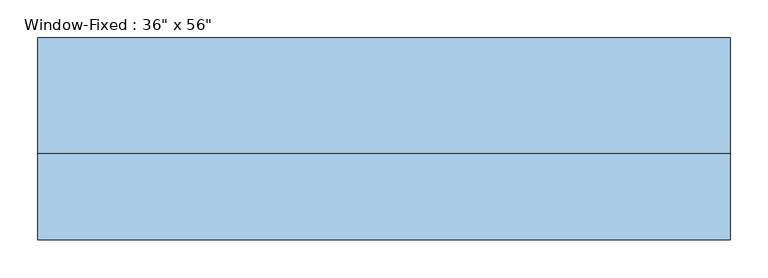
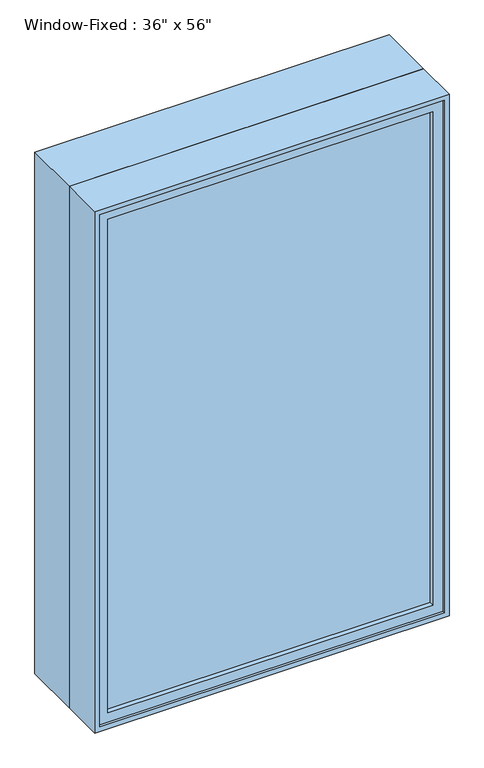
"""IFC4 building model written with IfcOpenShell, lengths in millimetres: window geometry."""

import ifcopenshell
import ifcopenshell.guid

model = None  # the IFC model being written
_history = None  # IfcOwnerHistory: only IFC2X3 demands one
_inside = {}  # id of a spatial element -> (the spatial element, [elements in it])
_under = {}  # id of a project, library or spatial element -> (it, [spatial elements below it])
_declared = {}  # id of a project -> (the project, [libraries it declares])
_typed = {}  # id of a type object -> (the type object, [elements of that type])
_made_of = {}  # id of a material, layer set ... -> (it, [elements and type objects made of it])


def new_model(schema):
    """Start an empty IFC model of exactly this schema.

    Asked for "IFC4X3", IfcOpenShell would pick the latest addendum, in which some entities
    have other attributes; the version numbers below select the first issue.
    IFC2X3 requires an IfcOwnerHistory on every rooted entity: one is made here for all.
    """
    global model, _history
    if schema == "IFC4X3":
        model = ifcopenshell.file(schema_version=(4, 3, 0, 0))
    else:
        model = ifcopenshell.file(schema=schema)
    _inside.clear()
    _under.clear()
    _declared.clear()
    _typed.clear()
    _made_of.clear()
    _history = None
    if model.schema == "IFC2X3":
        org = make("IfcOrganization", Name="unknown")
        user = make(
            "IfcPersonAndOrganization",
            ThePerson=make("IfcPerson", FamilyName="unknown"),
            TheOrganization=org,
        )
        app = make(
            "IfcApplication",
            ApplicationDeveloper=org,
            Version="unknown",
            ApplicationFullName="unknown",
            ApplicationIdentifier="unknown",
        )
        _history = make(
            "IfcOwnerHistory",
            OwningUser=user,
            OwningApplication=app,
            ChangeAction="ADDED",
            CreationDate=0,
        )
    return model


def make(cls, **values):
    """One entity of the class cls with the attributes given. An attribute that is None is left unset."""
    return model.create_entity(
        cls, **{name: value for name, value in values.items() if value is not None}
    )


def rooted(cls, **values):
    """An entity with a GlobalId (a new one), such as an element, a storey or a relation."""
    return make(cls, GlobalId=ifcopenshell.guid.new(), OwnerHistory=_history, **values)


def si_unit(unit_type, name, prefix=None):
    """IfcSIUnit, for example si_unit("LENGTHUNIT", "METRE", prefix="MILLI")."""
    return make("IfcSIUnit", UnitType=unit_type, Prefix=prefix, Name=name)


def assignment(units):
    """IfcUnitAssignment: the units of a project."""
    return None if units is None else make("IfcUnitAssignment", Units=units)


def point(xyz):
    """IfcCartesianPoint."""
    return None if xyz is None else make("IfcCartesianPoint", Coordinates=xyz)


def direction(xyz):
    """IfcDirection."""
    return None if xyz is None else make("IfcDirection", DirectionRatios=xyz)


def frame(location, z_axis=None, x_axis=None):
    """IfcAxis2Placement3D, a coordinate frame: its origin and axes. An axis left out is left unset."""
    return make(
        "IfcAxis2Placement3D",
        Location=point(location),
        Axis=direction(z_axis),
        RefDirection=direction(x_axis),
    )


def origin():
    """The frame at (0, 0, 0) with its axes left unset."""
    return frame((0.0, 0.0, 0.0))


def place(relative_to, where):
    """IfcLocalPlacement: puts the frame where relative to a parent placement (None: the world)."""
    return make(
        "IfcLocalPlacement", PlacementRelTo=relative_to, RelativePlacement=where
    )


def context(
    kind, dimensions, precision=None, world=None, true_north=None, identifier=None
):
    """IfcGeometricRepresentationContext, for example the 3D "Model" context."""
    return make(
        "IfcGeometricRepresentationContext",
        ContextIdentifier=identifier,
        ContextType=kind,
        CoordinateSpaceDimension=dimensions,
        Precision=precision,
        WorldCoordinateSystem=world,
        TrueNorth=true_north,
    )


def project(units=None, contexts=None):
    """IfcProject with its units and contexts."""
    return rooted(
        "IfcProject",
        Name="project",
        RepresentationContexts=contexts,
        UnitsInContext=assignment(units),
    )


def spatial(cls, under=None, at=None, **own):
    """A site, building, storey or space (cls), placed at a placement, below another one or the project."""
    s = rooted(cls, ObjectPlacement=at, **own)
    if under is not None:
        _under.setdefault(under.id(), (under, []))[1].append(s)
    return s


def polyline(points):
    """IfcPolyline through the points."""
    return make("IfcPolyline", Points=[point(p) for p in points])


def outline(outer, holes=None, kind="AREA"):
    """IfcArbitraryClosedProfileDef: a profile drawn as a closed curve; with holes, ...WithVoids."""
    if holes is None:
        return make("IfcArbitraryClosedProfileDef", ProfileType=kind, OuterCurve=outer)
    return make(
        "IfcArbitraryProfileDefWithVoids",
        ProfileType=kind,
        OuterCurve=outer,
        InnerCurves=holes,
    )


def extrude(swept, where, along, depth):
    """IfcExtrudedAreaSolid: the profile swept, set in the frame where, extruded along a direction by depth."""
    return make(
        "IfcExtrudedAreaSolid",
        SweptArea=swept,
        Position=where,
        ExtrudedDirection=direction(along),
        Depth=depth,
    )


def faces_of(points, faces, orient=None, outer=None):
    """IfcFace entities. A face is a list of loops; a loop is a list of indices into points, from 0.

    orient and outer hold one flag for each loop. By default every Orientation is true, the
    first loop of a face is its IfcFaceOuterBound and the others are IfcFaceBound.
    """
    made = []
    for i, loops in enumerate(faces):
        bounds = []
        for j, loop in enumerate(loops):
            is_outer = j == 0 if outer is None else outer[i][j]
            bounds.append(
                make(
                    "IfcFaceOuterBound" if is_outer else "IfcFaceBound",
                    Bound=make("IfcPolyLoop", Polygon=[points[k] for k in loop]),
                    Orientation=True if orient is None else orient[i][j],
                )
            )
        made.append(make("IfcFace", Bounds=bounds))
    return made


def faceted_brep(points, faces, orient=None, outer=None, voids=None):
    """IfcFacetedBrep: a solid bounded by flat faces; with voids (closed shells), ...WithVoids."""
    shared = [point(p) for p in points]
    hull = make("IfcClosedShell", CfsFaces=faces_of(shared, faces, orient, outer))
    if voids is None:
        return make("IfcFacetedBrep", Outer=hull)
    return make(
        "IfcFacetedBrepWithVoids",
        Outer=hull,
        Voids=[
            make(cls, CfsFaces=faces_of(shared, fs, o, b)) for cls, fs, o, b in voids
        ],
    )


def shape(context_of_items, identifier, shape_type, items):
    """IfcShapeRepresentation: the items that make up one representation, for example the "Body"."""
    return make(
        "IfcShapeRepresentation",
        ContextOfItems=context_of_items,
        RepresentationIdentifier=identifier,
        RepresentationType=shape_type,
        Items=items,
    )


def source(mapping_origin, context_of_items, identifier, shape_type, items):
    """IfcRepresentationMap: a shape defined once, which mapped items show again and again."""
    return make(
        "IfcRepresentationMap",
        MappingOrigin=mapping_origin,
        MappedRepresentation=shape(context_of_items, identifier, shape_type, items),
    )


def transform(
    local_origin,
    x_axis=None,
    y_axis=None,
    z_axis=None,
    scale=None,
    scale2=None,
    scale3=None,
    uniform=True,
):
    """IfcCartesianTransformationOperator3D, or its non-uniform kind. x_axis, y_axis, z_axis: its Axis1, 2, 3."""
    if uniform:
        return make(
            "IfcCartesianTransformationOperator3D",
            Axis1=direction(x_axis),
            Axis2=direction(y_axis),
            LocalOrigin=point(local_origin),
            Scale=scale,
            Axis3=direction(z_axis),
        )
    return make(
        "IfcCartesianTransformationOperator3DnonUniform",
        Axis1=direction(x_axis),
        Axis2=direction(y_axis),
        LocalOrigin=point(local_origin),
        Scale=scale,
        Axis3=direction(z_axis),
        Scale2=scale2,
        Scale3=scale3,
    )


def mapped(mapping_source, mapping_target):
    """IfcMappedItem: shows the shape of a source again, moved by a transform."""
    return make(
        "IfcMappedItem", MappingSource=mapping_source, MappingTarget=mapping_target
    )


def made_of(thing, what):
    """Note that an element or type object is made of a material, layer set ...; save() writes the relation."""
    if what is not None:
        _made_of.setdefault(what.id(), (what, []))[1].append(thing)
    return thing


def element(
    cls,
    number,
    at=None,
    inside=None,
    cuts=None,
    type_object=None,
    material=None,
    context=None,
    identifier="Body",
    shape_type=None,
    held_by="IfcProductDefinitionShape",
    body=None,
    shapes=None,
    **own,
):
    """One element of the class cls, such as IfcWall. Its Tag is "e" and its number.

    at: its placement. inside: the storey or other place that contains it. cuts: it is an
    opening in that element (IfcRelVoidsElement). A single representation is given by context,
    identifier, shape_type and body (its items); several are given by shapes. held_by: the class
    of the entity that holds the representations. save() writes the other relations.
    """
    e = rooted(cls, Tag="e%d" % number, ObjectPlacement=at, **own)
    if body is not None:
        shapes = [shape(context, identifier, shape_type, body)]
    if shapes is not None:
        e.Representation = make(held_by, Representations=shapes)
    if inside is not None:
        _inside.setdefault(inside.id(), (inside, []))[1].append(e)
    if cuts is not None:
        rooted(
            "IfcRelVoidsElement", RelatingBuildingElement=cuts, RelatedOpeningElement=e
        )
    if type_object is not None:
        _typed.setdefault(type_object.id(), (type_object, []))[1].append(e)
    return made_of(e, material)


def aggregate(whole, parts):
    """IfcRelAggregates: a whole, such as a stair, and the parts it consists of."""
    return rooted("IfcRelAggregates", RelatingObject=whole, RelatedObjects=parts)


def save(model, path):
    """Write the relations noted so far, then the file.

    IfcRelAggregates (storeys below a building ...), IfcRelContainedInSpatialStructure (elements
    in a storey), IfcRelDefinesByType, IfcRelAssociatesMaterial and IfcRelDeclares: one each for
    every whole, place, type object, material and project.
    """
    for whole, parts in _under.values():
        aggregate(whole, parts)
    for where, things in _inside.values():
        rooted(
            "IfcRelContainedInSpatialStructure",
            RelatedElements=things,
            RelatingStructure=where,
        )
    for kind, things in _typed.values():
        rooted("IfcRelDefinesByType", RelatedObjects=things, RelatingType=kind)
    for what, things in _made_of.values():
        rooted("IfcRelAssociatesMaterial", RelatedObjects=things, RelatingMaterial=what)
    for by, libraries in _declared.values():
        rooted("IfcRelDeclares", RelatingContext=by, RelatedDefinitions=libraries)
    model.write(path)


def window_66a382c3(model_context):
    return source(origin(), model_context, "Body", "SolidModel", [
        extrude(outline(polyline([(419.1, -79.375), (-419.1, -79.375), (-419.1, -73.025), (419.1, -73.025), (419.1, -79.375)])), frame((0.0, 0.0, 952.5), z_axis=(0.0, 0.0, 1.0), x_axis=(1.0, 0.0, 0.0)), (0.0, 0.0, 1.0), 1346.2),
        extrude(outline(polyline([(-419.1, -60.325), (419.1, -60.325), (419.1, -66.675), (-419.1, -66.675), (-419.1, -60.325)])), frame((0.0, 0.0, 952.5), z_axis=(0.0, 0.0, 1.0), x_axis=(1.0, 0.0, 0.0)), (0.0, 0.0, 1.0), 1346.2),
        extrude(outline(polyline([(927.1, -444.5), (927.1, 444.5), (2324.1, 444.5), (2324.1, -444.5), (927.1, -444.5)]), holes=[polyline([(952.5, 419.1), (952.5, -419.1), (2298.7, -419.1), (2298.7, 419.1), (952.5, 419.1)])]), frame((0.0, -92.075, 0.0), z_axis=(0.0, 1.0, 0.0), x_axis=(0.0, 0.0, 1.0)), (0.0, 0.0, 1.0), 44.45),
        extrude(outline(polyline([(2336.8, -457.2), (914.4, -457.2), (914.4, 457.2), (2336.8, 457.2), (2336.8, -457.2)]), holes=[polyline([(2324.1, 444.5), (927.1, 444.5), (927.1, -444.5), (2324.1, -444.5), (2324.1, 444.5)])]), frame((0.0, 15.875, 0.0), z_axis=(0.0, 1.0, 0.0), x_axis=(0.0, 0.0, 1.0)), (0.0, 0.0, 1.0), 152.4),
        faceted_brep([(457.2, 15.875, 2336.8), (-457.2, 15.875, 2336.8), (-457.2, -98.425, 2336.8), (457.2, -98.425, 2336.8), (-457.2, 15.875, 914.4), (-457.2, -98.425, 914.4), (457.2, 15.875, 914.4), (457.2, -98.425, 914.4), (425.45, 15.875, 2305.05), (-425.45, 15.875, 2305.05), (-425.45, 15.875, 946.15), (425.45, 15.875, 946.15), (-444.5, -98.425, 2324.1), (444.5, -98.425, 2324.1), (444.5, -98.425, 927.1), (-444.5, -98.425, 927.1), (425.45, -47.625, 2305.05), (-425.45, -47.625, 2305.05), (-444.5, -47.625, 2324.1), (444.5, -47.625, 2324.1), (-425.45, -47.625, 946.15), (-444.5, -47.625, 927.1), (425.45, -47.625, 946.15), (444.5, -47.625, 927.1)], [[[0, 1, 2, 3]], [[1, 4, 5, 2]], [[4, 6, 7, 5]], [[1, 0, 6, 4], [8, 9, 10, 11]], [[6, 0, 3, 7]], [[3, 2, 5, 7], [12, 13, 14, 15]], [[16, 17, 9, 8]], [[13, 12, 18, 19]], [[17, 20, 10, 9]], [[12, 15, 21, 18]], [[20, 22, 11, 10]], [[15, 14, 23, 21]], [[22, 16, 8, 11]], [[19, 18, 21, 23], [17, 16, 22, 20]], [[14, 13, 19, 23]]]),
    ])


if __name__ == "__main__":
    model = new_model("IFC4")
    model_context = context("Model", 3, world=origin())
    ifc_project = project(units=[si_unit("LENGTHUNIT", "METRE", prefix="MILLI")], contexts=[model_context])
    site = spatial("IfcSite", under=ifc_project)
    building = spatial("IfcBuilding", under=site)
    placement = place(None, origin())
    window_shape = window_66a382c3(model_context)
    element("IfcWindow", 1, ObjectType="Window-Fixed : 36\" x 56\"", at=placement, inside=building, context=model_context, shape_type="MappedRepresentation", body=[
        mapped(window_shape, transform((0.0, 0.0, 0.0), x_axis=(1.0, 0.0, 0.0), y_axis=(0.0, 1.0, 0.0), z_axis=(0.0, 0.0, 1.0))),
    ])
    save(model, "model.ifc")

# Revit data of these elements
# Type "Window-Fixed : 36\" x 56\""
#   Type Mark = "22"
#   Fire Rating = "0.5h"
#   Assembly Code = "B2020100"
#   Analytic Construction = "Double glazing - domestic"
#   Window Inset [instance default] = 0' - 0"
#   Wall Thickness [instance default] = 0' - 6"
#   Visual Light Transmittance = 0.81
#   Thermal Resistance (R) = 1.8146 (h·ft²·°F)/BTU
#   Solar Heat Gain Coefficient = 0.76
#   Rough Width = 3' - 0 1/2"
#   Rough Height = 4' - 8 1/2"
#   Interior Wall Closure [instance default] = 0' - 2 1/4"
#   Height = 4' - 8"
#   Heat Transfer Coefficient (U) = 0.5511 BTU/(h·ft²·°F)
#   Frame Extension [instance default] = 0' - 0 1/4"
#   Exterior Wall Closure [instance default] = 0' - 1 1/4"
#   Extension Jamb [instance default] = 0' - 2 1/4"
#   Default Sill Height = 3' - 0"
#   Width = 3' - 0"
#   Muntin Visibility = yes
#   Interior Trim Visibility [instance default] = yes
#   Exterior Trim Visibility [instance default] = yes
#   Extension Jamb Visibility [instance default] = yes
#   Muntin Pattern = Muntin Pattern_2x2 : Muntin Pattern_2x2
#   Interior Trim Material = Wood - Stained
#   Interior Trim = Trim-Window-Interior-Flat : Picture Frame
#   Interior Frame Material = Wood - Stained
#   Glass Panel Material = Glass
#   Exterior Trim Material = Clad - White
#   Exterior Trim = Trim-Window-Exterior-Flat : with Sill
#   Exterior Frame Material = Clad - White
#   Wall Closure = (empty or 0)
# Element 1 (IfcWindow, "Window-Fixed : 36\" x 56\"")
#   Window Inset = 0' - 3 1/2"
#   Wall Thickness = 1' - 1 1/4"
#   Exterior Wall Closure = 0' - 5 1/2"
#   Extension Jamb = 0' - 6"
#   Exterior Trim Visibility = no
#   Materials on its faces: "Wood - Stained", "Glass", "Clad - White"
# Materials
#   "Wood - Stained": class "Wood", colour RGB 224 178 126, transparency 0, Cost = 0
#   "Glass": class "Glass", colour RGB 0 128 192, transparency 0.75, Description = "Soda Lime Glass", Cost = 0
#   "Clad - White": class "Wood", colour RGB 242 242 238, transparency 0, Cost = 0
